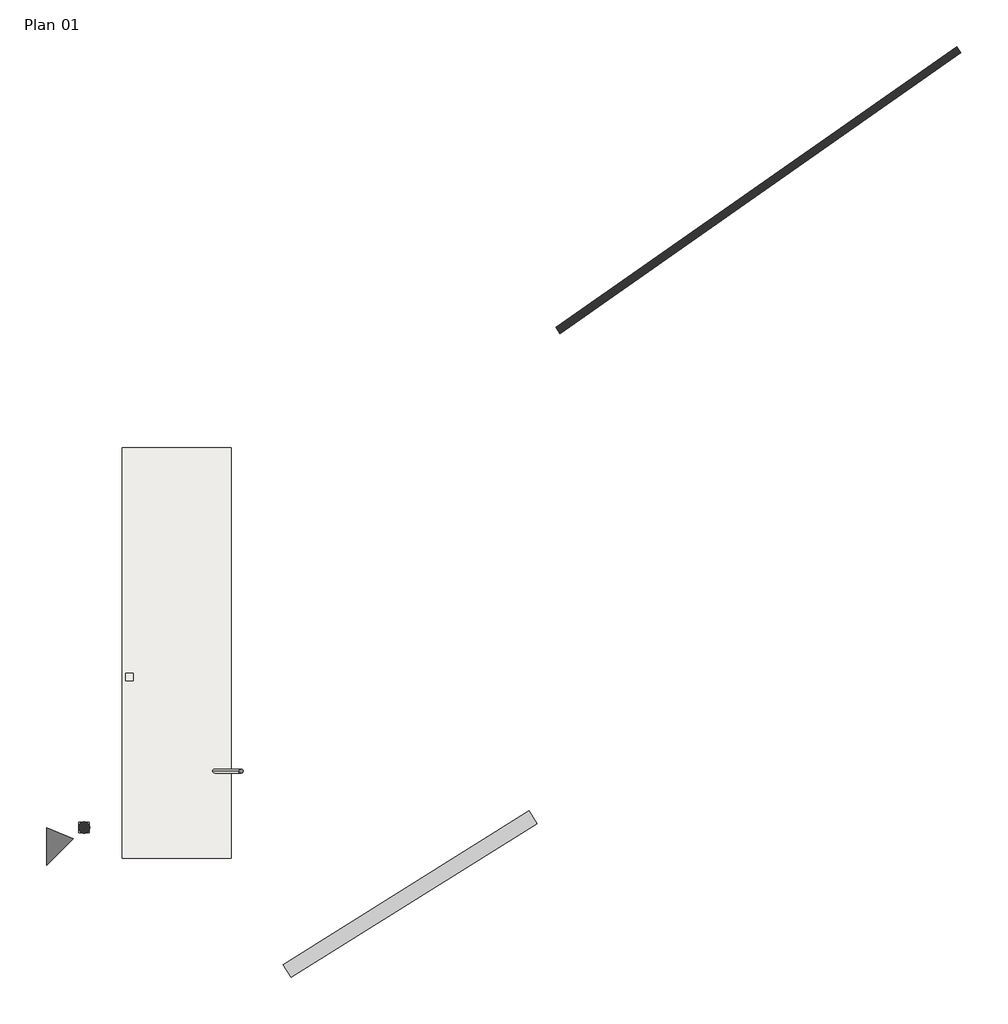
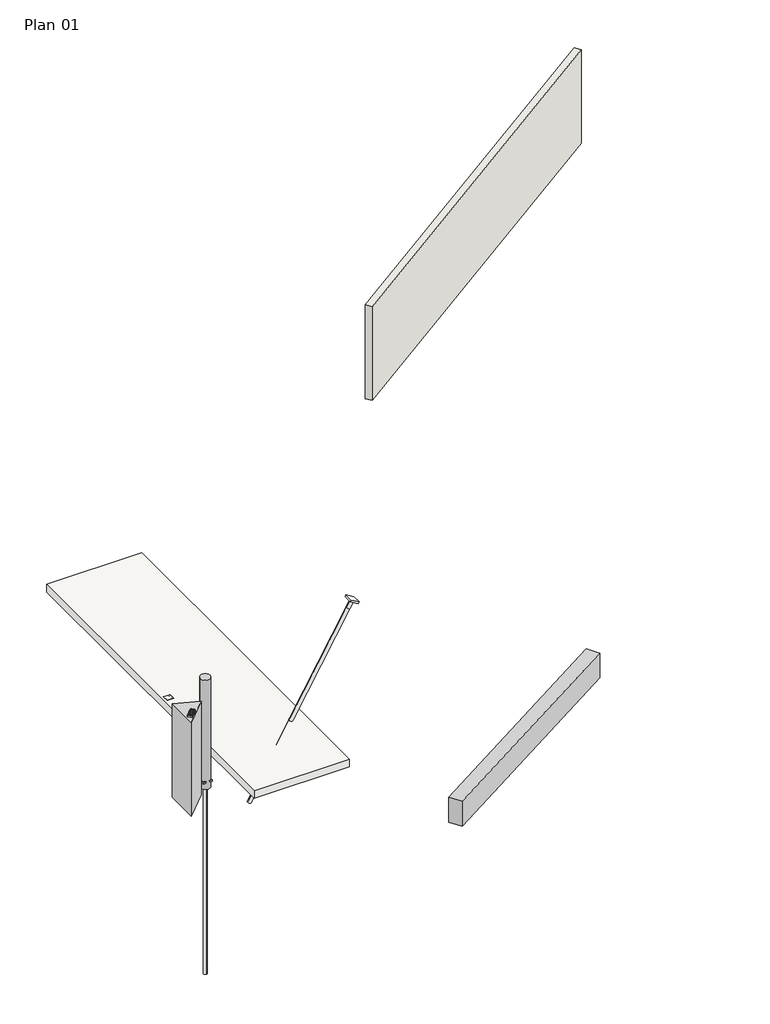
# One storey: 4 slabs, 1 beam, 1 column, 1 geographic element, 1 wall.
"""IFC4 building model written with IfcOpenShell, lengths in millimetres."""

import ifcopenshell
import ifcopenshell.guid

model = None  # the IFC model being written
_history = None  # IfcOwnerHistory: only IFC2X3 demands one
_inside = {}  # id of a spatial element -> (the spatial element, [elements in it])
_under = {}  # id of a project, library or spatial element -> (it, [spatial elements below it])
_declared = {}  # id of a project -> (the project, [libraries it declares])
_typed = {}  # id of a type object -> (the type object, [elements of that type])
_made_of = {}  # id of a material, layer set ... -> (it, [elements and type objects made of it])


def new_model(schema):
    """Start an empty IFC model of exactly this schema.

    Asked for "IFC4X3", IfcOpenShell would pick the latest addendum, in which some entities
    have other attributes; the version numbers below select the first issue.
    IFC2X3 requires an IfcOwnerHistory on every rooted entity: one is made here for all.
    """
    global model, _history
    if schema == "IFC4X3":
        model = ifcopenshell.file(schema_version=(4, 3, 0, 0))
    else:
        model = ifcopenshell.file(schema=schema)
    _inside.clear()
    _under.clear()
    _declared.clear()
    _typed.clear()
    _made_of.clear()
    _history = None
    if model.schema == "IFC2X3":
        org = make("IfcOrganization", Name="unknown")
        user = make(
            "IfcPersonAndOrganization",
            ThePerson=make("IfcPerson", FamilyName="unknown"),
            TheOrganization=org,
        )
        app = make(
            "IfcApplication",
            ApplicationDeveloper=org,
            Version="unknown",
            ApplicationFullName="unknown",
            ApplicationIdentifier="unknown",
        )
        _history = make(
            "IfcOwnerHistory",
            OwningUser=user,
            OwningApplication=app,
            ChangeAction="ADDED",
            CreationDate=0,
        )
    return model


def make(cls, **values):
    """One entity of the class cls with the attributes given. An attribute that is None is left unset."""
    return model.create_entity(
        cls, **{name: value for name, value in values.items() if value is not None}
    )


def rooted(cls, **values):
    """An entity with a GlobalId (a new one), such as an element, a storey or a relation."""
    return make(cls, GlobalId=ifcopenshell.guid.new(), OwnerHistory=_history, **values)


def si_unit(unit_type, name, prefix=None):
    """IfcSIUnit, for example si_unit("LENGTHUNIT", "METRE", prefix="MILLI")."""
    return make("IfcSIUnit", UnitType=unit_type, Prefix=prefix, Name=name)


def assignment(units):
    """IfcUnitAssignment: the units of a project."""
    return None if units is None else make("IfcUnitAssignment", Units=units)


def point(xyz):
    """IfcCartesianPoint."""
    return None if xyz is None else make("IfcCartesianPoint", Coordinates=xyz)


def direction(xyz):
    """IfcDirection."""
    return None if xyz is None else make("IfcDirection", DirectionRatios=xyz)


def frame(location, z_axis=None, x_axis=None):
    """IfcAxis2Placement3D, a coordinate frame: its origin and axes. An axis left out is left unset."""
    return make(
        "IfcAxis2Placement3D",
        Location=point(location),
        Axis=direction(z_axis),
        RefDirection=direction(x_axis),
    )


def frame_2d(location, x_axis=None):
    """IfcAxis2Placement2D, a coordinate frame in the plane: its origin and x axis."""
    return make(
        "IfcAxis2Placement2D", Location=point(location), RefDirection=direction(x_axis)
    )


def origin():
    """The frame at (0, 0, 0) with its axes left unset."""
    return frame((0.0, 0.0, 0.0))


def origin_with_axes():
    """The frame at (0, 0, 0) with the z axis (0, 0, 1) and the x axis (1, 0, 0) written out."""
    return frame((0.0, 0.0, 0.0), z_axis=(0.0, 0.0, 1.0), x_axis=(1.0, 0.0, 0.0))


def origin_2d():
    """The frame at (0, 0) in the plane with its x axis left unset."""
    return frame_2d((0.0, 0.0))


def place(relative_to, where):
    """IfcLocalPlacement: puts the frame where relative to a parent placement (None: the world)."""
    return make(
        "IfcLocalPlacement", PlacementRelTo=relative_to, RelativePlacement=where
    )


def context(
    kind, dimensions, precision=None, world=None, true_north=None, identifier=None
):
    """IfcGeometricRepresentationContext, for example the 3D "Model" context."""
    return make(
        "IfcGeometricRepresentationContext",
        ContextIdentifier=identifier,
        ContextType=kind,
        CoordinateSpaceDimension=dimensions,
        Precision=precision,
        WorldCoordinateSystem=world,
        TrueNorth=true_north,
    )


def project(units=None, contexts=None):
    """IfcProject with its units and contexts."""
    return rooted(
        "IfcProject",
        Name="project",
        RepresentationContexts=contexts,
        UnitsInContext=assignment(units),
    )


def spatial(cls, under=None, at=None, **own):
    """A site, building, storey or space (cls), placed at a placement, below another one or the project."""
    s = rooted(cls, ObjectPlacement=at, **own)
    if under is not None:
        _under.setdefault(under.id(), (under, []))[1].append(s)
    return s


def polyline(points):
    """IfcPolyline through the points."""
    return make("IfcPolyline", Points=[point(p) for p in points])


def circle_curve(where, radius):
    """IfcCircle in the frame where."""
    return make("IfcCircle", Position=where, Radius=radius)


def trimmed(basis, trim1, trim2, sense, master):
    """IfcTrimmedCurve: the piece of a basis curve between two trims."""
    return make(
        "IfcTrimmedCurve",
        BasisCurve=basis,
        Trim1=trim1,
        Trim2=trim2,
        SenseAgreement=sense,
        MasterRepresentation=master,
    )


def segment(curve, same_sense, transition):
    """IfcCompositeCurveSegment."""
    return make(
        "IfcCompositeCurveSegment",
        Transition=transition,
        SameSense=same_sense,
        ParentCurve=curve,
    )


def composite_curve(segments, self_intersect=None):
    """IfcCompositeCurve: segments joined end to end."""
    return make("IfcCompositeCurve", Segments=segments, SelfIntersect=self_intersect)


def outline(outer, holes=None, kind="AREA"):
    """IfcArbitraryClosedProfileDef: a profile drawn as a closed curve; with holes, ...WithVoids."""
    if holes is None:
        return make("IfcArbitraryClosedProfileDef", ProfileType=kind, OuterCurve=outer)
    return make(
        "IfcArbitraryProfileDefWithVoids",
        ProfileType=kind,
        OuterCurve=outer,
        InnerCurves=holes,
    )


def extrude(swept, where, along, depth):
    """IfcExtrudedAreaSolid: the profile swept, set in the frame where, extruded along a direction by depth."""
    return make(
        "IfcExtrudedAreaSolid",
        SweptArea=swept,
        Position=where,
        ExtrudedDirection=direction(along),
        Depth=depth,
    )


def faces_of(points, faces, orient=None, outer=None):
    """IfcFace entities. A face is a list of loops; a loop is a list of indices into points, from 0.

    orient and outer hold one flag for each loop. By default every Orientation is true, the
    first loop of a face is its IfcFaceOuterBound and the others are IfcFaceBound.
    """
    made = []
    for i, loops in enumerate(faces):
        bounds = []
        for j, loop in enumerate(loops):
            is_outer = j == 0 if outer is None else outer[i][j]
            bounds.append(
                make(
                    "IfcFaceOuterBound" if is_outer else "IfcFaceBound",
                    Bound=make("IfcPolyLoop", Polygon=[points[k] for k in loop]),
                    Orientation=True if orient is None else orient[i][j],
                )
            )
        made.append(make("IfcFace", Bounds=bounds))
    return made


def faceted_brep(points, faces, orient=None, outer=None, voids=None):
    """IfcFacetedBrep: a solid bounded by flat faces; with voids (closed shells), ...WithVoids."""
    shared = [point(p) for p in points]
    hull = make("IfcClosedShell", CfsFaces=faces_of(shared, faces, orient, outer))
    if voids is None:
        return make("IfcFacetedBrep", Outer=hull)
    return make(
        "IfcFacetedBrepWithVoids",
        Outer=hull,
        Voids=[
            make(cls, CfsFaces=faces_of(shared, fs, o, b)) for cls, fs, o, b in voids
        ],
    )


def shape(context_of_items, identifier, shape_type, items):
    """IfcShapeRepresentation: the items that make up one representation, for example the "Body"."""
    return make(
        "IfcShapeRepresentation",
        ContextOfItems=context_of_items,
        RepresentationIdentifier=identifier,
        RepresentationType=shape_type,
        Items=items,
    )


def source(mapping_origin, context_of_items, identifier, shape_type, items):
    """IfcRepresentationMap: a shape defined once, which mapped items show again and again."""
    return make(
        "IfcRepresentationMap",
        MappingOrigin=mapping_origin,
        MappedRepresentation=shape(context_of_items, identifier, shape_type, items),
    )


def transform(
    local_origin,
    x_axis=None,
    y_axis=None,
    z_axis=None,
    scale=None,
    scale2=None,
    scale3=None,
    uniform=True,
):
    """IfcCartesianTransformationOperator3D, or its non-uniform kind. x_axis, y_axis, z_axis: its Axis1, 2, 3."""
    if uniform:
        return make(
            "IfcCartesianTransformationOperator3D",
            Axis1=direction(x_axis),
            Axis2=direction(y_axis),
            LocalOrigin=point(local_origin),
            Scale=scale,
            Axis3=direction(z_axis),
        )
    return make(
        "IfcCartesianTransformationOperator3DnonUniform",
        Axis1=direction(x_axis),
        Axis2=direction(y_axis),
        LocalOrigin=point(local_origin),
        Scale=scale,
        Axis3=direction(z_axis),
        Scale2=scale2,
        Scale3=scale3,
    )


def mapped(mapping_source, mapping_target):
    """IfcMappedItem: shows the shape of a source again, moved by a transform."""
    return make(
        "IfcMappedItem", MappingSource=mapping_source, MappingTarget=mapping_target
    )


def made_of(thing, what):
    """Note that an element or type object is made of a material, layer set ...; save() writes the relation."""
    if what is not None:
        _made_of.setdefault(what.id(), (what, []))[1].append(thing)
    return thing


def element(
    cls,
    number,
    at=None,
    inside=None,
    cuts=None,
    type_object=None,
    material=None,
    context=None,
    identifier="Body",
    shape_type=None,
    held_by="IfcProductDefinitionShape",
    body=None,
    shapes=None,
    **own,
):
    """One element of the class cls, such as IfcWall. Its Tag is "e" and its number.

    at: its placement. inside: the storey or other place that contains it. cuts: it is an
    opening in that element (IfcRelVoidsElement). A single representation is given by context,
    identifier, shape_type and body (its items); several are given by shapes. held_by: the class
    of the entity that holds the representations. save() writes the other relations.
    """
    e = rooted(cls, Tag="e%d" % number, ObjectPlacement=at, **own)
    if body is not None:
        shapes = [shape(context, identifier, shape_type, body)]
    if shapes is not None:
        e.Representation = make(held_by, Representations=shapes)
    if inside is not None:
        _inside.setdefault(inside.id(), (inside, []))[1].append(e)
    if cuts is not None:
        rooted(
            "IfcRelVoidsElement", RelatingBuildingElement=cuts, RelatedOpeningElement=e
        )
    if type_object is not None:
        _typed.setdefault(type_object.id(), (type_object, []))[1].append(e)
    return made_of(e, material)


def aggregate(whole, parts):
    """IfcRelAggregates: a whole, such as a stair, and the parts it consists of."""
    return rooted("IfcRelAggregates", RelatingObject=whole, RelatedObjects=parts)


def save(model, path):
    """Write the relations noted so far, then the file.

    IfcRelAggregates (storeys below a building ...), IfcRelContainedInSpatialStructure (elements
    in a storey), IfcRelDefinesByType, IfcRelAssociatesMaterial and IfcRelDeclares: one each for
    every whole, place, type object, material and project.
    """
    for whole, parts in _under.values():
        aggregate(whole, parts)
    for where, things in _inside.values():
        rooted(
            "IfcRelContainedInSpatialStructure",
            RelatedElements=things,
            RelatingStructure=where,
        )
    for kind, things in _typed.values():
        rooted("IfcRelDefinesByType", RelatedObjects=things, RelatingType=kind)
    for what, things in _made_of.values():
        rooted("IfcRelAssociatesMaterial", RelatedObjects=things, RelatingMaterial=what)
    for by, libraries in _declared.values():
        rooted("IfcRelDeclares", RelatingContext=by, RelatedDefinitions=libraries)
    model.write(path)


def plane_surface(at):
    """IfcPlane: the flat surface through the origin of the frame at, square to its z axis."""
    return make("IfcPlane", Position=at)


def cylinder_surface(at, radius):
    """IfcCylindricalSurface: all points at the distance radius from the z axis of the frame at."""
    return make("IfcCylindricalSurface", Position=at, Radius=radius)


def advanced_brep(points, edges, surfaces, faces):
    """IfcAdvancedBrep: a solid bounded by faces that lie on surfaces and meet in shared edges.

    An edge is (start, end): straight between two places in points (the first is 0);
    or (start, end, curve); or (start, end, curve, False) where it runs against its curve.
    A face is (place in surfaces, loops), or (place, loops, False) where it looks against
    its surface's normal. A loop lists edges by number (the first is 1), with a minus sign
    where the edge is run from its end to its start. The first loop is the outer one.
    """
    corners = [point(p) for p in points]
    vertices = [make("IfcVertexPoint", VertexGeometry=c) for c in corners]
    made = []
    for start, end, *more in edges:
        made.append(
            make(
                "IfcEdgeCurve",
                EdgeStart=vertices[start],
                EdgeEnd=vertices[end],
                EdgeGeometry=more[0] if more else make("IfcPolyline", Points=[corners[start], corners[end]]),
                SameSense=more[1] if len(more) > 1 else True,
            )
        )
    hull = []
    for where, loops, *sense in faces:
        bounds = []
        for j, loop in enumerate(loops):
            ring = [make("IfcOrientedEdge", EdgeElement=made[abs(k) - 1], Orientation=k > 0) for k in loop]
            bounds.append(
                make(
                    "IfcFaceOuterBound" if j == 0 else "IfcFaceBound",
                    Bound=make("IfcEdgeLoop", EdgeList=ring),
                    Orientation=True,
                )
            )
        hull.append(make("IfcAdvancedFace", Bounds=bounds, FaceSurface=surfaces[where], SameSense=sense[0] if sense else True))
    return make("IfcAdvancedBrep", Outer=make("IfcClosedShell", CfsFaces=hull))


def beam_400x800mm_1e0f6873(model_context):
    return source(origin(), model_context, "Body", "SweptSolid", [
        extrude(outline(polyline([(3850.0, 200.0), (3850.0, -200.0), (-3850.0, -200.0), (-3850.0, 200.0), (3850.0, 200.0)])), frame((0.0, 0.0, -400.0), z_axis=(0.0, 0.0, 1.0), x_axis=(1.0, 0.0, 0.0)), (0.0, 0.0, 1.0), 800.0),
    ])


def column_bdfed939(model_context):
    return source(origin(), model_context, "Body", "SweptSolid", [
        extrude(outline(composite_curve([segment(trimmed(circle_curve(origin_2d(), 150.0), [point((-150.0, 0.0))], [point((150.0, 0.0))], False, "CARTESIAN"), True, "CONTINUOUS"), segment(trimmed(circle_curve(origin_2d(), 150.0), [point((150.0, 0.0))], [point((-150.0, 0.0))], False, "CARTESIAN"), True, "CONTINUOUS")], self_intersect=False)), origin_with_axes(), (0.0, 0.0, 1.0), 3500.0),
    ])


def rib_79407f03(model_context):
    return source(origin(), model_context, "Body", "SweptSolid", [
        extrude(outline(polyline([(0.0, 1000.0), (707.1067812, 707.1067812), (0.0, 0.0), (0.0, 1000.0)])), origin_with_axes(), (0.0, 0.0, 1.0), 3000.0),
        extrude(outline(polyline([(25.1140775, 0.0), (25.1140775, -200.9126203), (-61.4608186, -200.9126203), (-84.7293549, -199.5575883), (-101.658058, -195.4924922), (-114.0311558, -187.9876995), (-123.6328759, -176.3135776), (-129.7948993, -161.837421), (-131.8489071, -145.9265248), (-128.4459986, -126.1344734), (-118.2372733, -109.7269364), (-100.9161627, -97.6971952), (-76.1760985, -91.0385311), (-90.4499198, -80.2963768), (-110.806057, -54.4465353), (-144.307844, 0.0), (-115.1225391, 0.0), (-88.9783919, -41.6442419), (-70.0937828, -69.210866), (-56.8255055, -82.2338887), (-44.8816034, -87.0163546), (-30.3134764, -87.8992714), (0.0, -87.8992714), (0.0, 0.0), (25.1140775, 0.0)]), holes=[polyline([(0.0, -113.0133489), (-56.2123689, -113.0133489), (-84.882639, -116.5695415), (-94.3126808, -121.1925919), (-101.1675487, -127.9493579), (-106.7348295, -144.994557), (-104.0799478, -157.2450275), (-96.1153027, -167.1165277), (-82.4116983, -173.628039), (-62.5399392, -175.7985428), (0.0, -175.7985428), (0.0, -113.0133489)])]), frame((497.5715471, 793.899117, 2400.0), z_axis=(0.38268343236508784, 0.9238795325112875, 0.0), x_axis=(0.9238795325112875, -0.38268343236508784, 0.0)), (0.0, 0.0, 1.0), 50.0),
        extrude(outline(polyline([(328.1863632, 918.1803674), (351.3887454, 908.569626), (332.2545738, 862.3756494), (309.0521916, 871.9863908), (328.1863632, 918.1803674)])), frame((0.0, 0.0, 2400.0), z_axis=(0.0, 0.0, 1.0), x_axis=(1.0, 0.0, 0.0)), (0.0, 0.0, 1.0), 200.9126203),
        extrude(outline(polyline([(76.0779965, 0.0), (76.0779965, -200.9126203), (-0.5886112, -200.9126203), (-21.6743809, -199.434961), (-38.1371002, -195.0019829), (-50.7554526, -187.5033216), (-60.3081217, -176.8286123), (-66.3229924, -164.2715736), (-68.3279493, -151.1259236), (-66.6418234, -139.0287373), (-61.583446, -127.6550523), (-53.1160287, -117.7038444), (-41.2027834, -109.8740892), (-55.4336854, -102.4428729), (-65.948979, -91.1366329), (-72.4420962, -76.703396), (-74.6064686, -59.8911888), (-68.6958312, -32.8886504), (-54.0541278, -13.6606848), (-32.2019373, -3.4580908), (0.0, 0.0), (76.0779965, 0.0)]), holes=[polyline([(50.9639191, -119.2918683), (5.101297, -119.2918683), (-21.6805123, -121.4501093), (-37.7937437, -130.7452611), (-43.2138717, -147.1037471), (-38.1616256, -163.4867587), (-23.6916005, -173.1743179), (8.5839132, -175.7985428), (50.9639191, -175.7985428), (50.9639191, -119.2918683)]), polyline([(50.9639191, -25.1140775), (-0.5395603, -25.1140775), (-19.1789147, -26.0950962), (-34.9487895, -31.5642752), (-45.3966382, -42.7233624), (-49.4923911, -59.6459342), (-44.6853997, -79.1682054), (-38.3884862, -86.2254083), (-29.1117286, -90.8178019), (1.9129864, -94.1777908), (50.9639191, -94.1777908), (50.9639191, -25.1140775)])]), frame((192.3605232, 920.3216624, 2400.0), z_axis=(0.38268343236508784, 0.9238795325112875, 0.0), x_axis=(0.9238795325112875, -0.38268343236508784, 0.0)), (0.0, 0.0, 1.0), 50.0),
        extrude(outline(polyline([(142.0846737, 166.9156415), (34.8288922, 272.7551681), (80.4360125, 318.9725642), (104.5051668, 337.5762862), (115.0296187, 340.2280985), (126.319893, 339.2040535), (137.2940026, 334.8676564), (146.8699607, 327.5824121), (155.6431762, 315.3394631), (159.0243303, 301.2462182), (156.3216686, 285.6622725), (146.8434364, 268.9472211), (160.0974204, 270.9082992), (184.6206627, 268.1577423), (231.3350949, 257.3603361), (215.9604566, 241.7799674), (179.9563975, 249.7610286), (155.2918548, 254.2015408), (141.3499598, 253.9788127), (132.5049003, 250.1220185), (124.3591622, 242.810042), (108.3902102, 226.627407), (155.3146145, 180.3226141), (142.0846737, 166.9156415)]), holes=[polyline([(94.9832375, 239.8573479), (124.595566, 269.8659235), (137.8004388, 287.0447247), (140.3041941, 301.7331255), (134.1375442, 313.6844846), (126.1991419, 318.7206668), (116.7335855, 319.6690426), (106.0384872, 315.7836943), (94.4114592, 306.3187042), (61.4658058, 272.9322), (94.9832375, 239.8573479)])]), frame((0.0, 0.0, 3000.0), z_axis=(0.0, 0.0, 1.0), x_axis=(1.0, 0.0, 0.0)), (0.0, 0.0, 1.0), 50.0),
        extrude(outline(polyline([(249.577943, 275.8472945), (142.3221615, 381.6868212), (155.5521023, 395.0937938), (262.8078838, 289.2542672), (249.577943, 275.8472945)])), frame((0.0, 0.0, 3000.0), z_axis=(0.0, 0.0, 1.0), x_axis=(1.0, 0.0, 0.0)), (0.0, 0.0, 1.0), 50.0),
        extrude(outline(polyline([(289.2677655, 316.0682125), (182.011984, 421.9077392), (222.3994792, 462.8356656), (245.3351431, 479.7669736), (255.9855205, 482.5529434), (266.7164256, 482.0291974), (284.6624197, 472.770508), (293.6392157, 456.8056927), (292.3950501, 436.5587187), (303.8589035, 440.2410662), (315.4340515, 439.898524), (326.559667, 435.7614887), (336.6749229, 428.0603568), (347.9763498, 410.6802344), (350.5279044, 392.7346911), (344.4628882, 375.6943903), (329.3451839, 356.681913), (289.2677655, 316.0682125)]), holes=[polyline([(238.8145861, 392.3174042), (262.9747319, 416.8008406), (275.9310618, 432.2350681), (279.4572615, 445.7336312), (273.5796894, 457.2446776), (262.1722425, 463.178041), (249.3778877, 460.5566667), (230.9744227, 444.7090375), (208.6488975, 422.0847711), (238.8145861, 392.3174042)]), polyline([(289.0907336, 342.7051261), (316.2224482, 370.1998943), (325.5178351, 380.6671764), (330.9056251, 391.9669422), (330.4522875, 403.4229905), (323.5759095, 414.5241854), (310.6217897, 422.2422189), (296.1986213, 420.0652601), (278.0612869, 405.2729569), (252.2215587, 379.0874633), (289.0907336, 342.7051261)])]), frame((0.0, 0.0, 3000.0), z_axis=(0.0, 0.0, 1.0), x_axis=(1.0, 0.0, 0.0)), (0.0, 0.0, 1.0), 50.0),
    ])


def slab_200x200_02b47a6d(model_context):
    return source(origin(), model_context, "Body", "SweptSolid", [
        extrude(outline(composite_curve([segment(trimmed(circle_curve(frame_2d((269.1096391, -214.6158832)), 6.0), [point((263.1096391, -214.6158832))], [point((275.1096391, -214.6158832))], False, "CARTESIAN"), True, "CONTINUOUS"), segment(trimmed(circle_curve(frame_2d((269.1096391, -214.6158832)), 6.0), [point((275.1096391, -214.6158832))], [point((263.1096391, -214.6158832))], False, "CARTESIAN"), True, "CONTINUOUS")], self_intersect=False)), frame((0.0, 0.0, -200.0), z_axis=(0.0, 0.0, 1.0), x_axis=(1.0, 0.0, 0.0)), (0.0, 0.0, 1.0), 185.0),
        extrude(outline(composite_curve([segment(trimmed(circle_curve(frame_2d((369.1096391, -214.6158832)), 6.0), [point((363.1096391, -214.6158832))], [point((375.1096391, -214.6158832))], False, "CARTESIAN"), True, "CONTINUOUS"), segment(trimmed(circle_curve(frame_2d((369.1096391, -214.6158832)), 6.0), [point((375.1096391, -214.6158832))], [point((363.1096391, -214.6158832))], False, "CARTESIAN"), True, "CONTINUOUS")], self_intersect=False)), frame((0.0, 0.0, -200.0), z_axis=(0.0, 0.0, 1.0), x_axis=(1.0, 0.0, 0.0)), (0.0, 0.0, 1.0), 185.0),
        extrude(outline(composite_curve([segment(trimmed(circle_curve(frame_2d((369.1096391, -314.6158832)), 6.0), [point((363.1096391, -314.6158832))], [point((375.1096391, -314.6158832))], False, "CARTESIAN"), True, "CONTINUOUS"), segment(trimmed(circle_curve(frame_2d((369.1096391, -314.6158832)), 6.0), [point((375.1096391, -314.6158832))], [point((363.1096391, -314.6158832))], False, "CARTESIAN"), True, "CONTINUOUS")], self_intersect=False)), frame((0.0, 0.0, -200.0), z_axis=(0.0, 0.0, 1.0), x_axis=(1.0, 0.0, 0.0)), (0.0, 0.0, 1.0), 185.0),
        extrude(outline(composite_curve([segment(trimmed(circle_curve(frame_2d((269.1096391, -314.6158832)), 6.0), [point((263.1096391, -314.6158832))], [point((275.1096391, -314.6158832))], False, "CARTESIAN"), True, "CONTINUOUS"), segment(trimmed(circle_curve(frame_2d((269.1096391, -314.6158832)), 6.0), [point((275.1096391, -314.6158832))], [point((263.1096391, -314.6158832))], False, "CARTESIAN"), True, "CONTINUOUS")], self_intersect=False)), frame((0.0, 0.0, -200.0), z_axis=(0.0, 0.0, 1.0), x_axis=(1.0, 0.0, 0.0)), (0.0, 0.0, 1.0), 185.0),
        extrude(outline(polyline([(419.1096391, -164.6158832), (419.1096391, -364.6158832), (219.1096391, -364.6158832), (219.1096391, -164.6158832), (419.1096391, -164.6158832)])), frame((0.0, 0.0, -15.0), z_axis=(0.0, 0.0, 1.0), x_axis=(1.0, 0.0, 0.0)), (0.0, 0.0, 1.0), 15.0),
    ])


model = new_model("IFC4")

# Units and contexts
model_context = context("Model", 3, world=origin())
ifc_project = project(units=[si_unit("LENGTHUNIT", "METRE", prefix="MILLI")], contexts=[model_context])

# Site, building, storey
site = spatial("IfcSite", under=ifc_project)
building = spatial("IfcBuilding", under=site)
storey = spatial("IfcBuildingStorey", under=building, Name="Plan 01", Elevation=0.0)

# Beam
placement = place(None, origin())
beam_400x800mm_shape = beam_400x800mm_1e0f6873(model_context)
element("IfcBeam", 1, ObjectType="S-Frame_CastInPlace_Rectangular : 400x800mm", at=placement, inside=storey, context=model_context, shape_type="MappedRepresentation", body=[
    mapped(beam_400x800mm_shape, transform((9658.2803674, -768.6963803, -400.0), x_axis=(0.8480480961564263, 0.5299192642332045, 0.0), y_axis=(-0.5299192642332045, 0.8480480961564263, 0.0), z_axis=(0.0, 0.0, 1.0))),
])

# Column
column_shape = column_bdfed939(model_context)
element("IfcColumn", 2, ObjectType="S-Column_CastInPlace_Round : Ø300", at=placement, inside=storey, context=model_context, shape_type="MappedRepresentation", body=[
    mapped(column_shape, transform((1000.0, 1000.0, 0.0), x_axis=(1.0, 0.0, 0.0), y_axis=(0.0, 1.0, 0.0), z_axis=(0.0, 0.0, 1.0))),
])

# Geographic element
rib_shape = rib_79407f03(model_context)
element("IfcGeographicElement", 3, ObjectType="NO_Origo : RIB", at=placement, inside=storey, context=model_context, shape_type="MappedRepresentation", body=[
    mapped(rib_shape, transform((0.0, 0.0, 0.0), x_axis=(1.0, 0.0, 0.0), y_axis=(0.0, 1.0, 0.0), z_axis=(0.0, 0.0, 1.0))),
])

# Slabs
element("IfcSlab", 4, ObjectType="Betongdekke 250mm", at=placement, inside=storey, context=model_context, shape_type="Brep", body=[
    faceted_brep([(2011.4794189, 11088.1813587, -250.0), (4900.8131513, 11088.1813587, -250.0), (4900.8131513, 182.737712, -250.0), (2011.4794189, 182.737712, -250.0), (4900.8131513, 11088.1813587, 0.0), (2011.4794189, 11088.1813587, 0.0), (2011.4794189, 182.737712, 0.0), (4900.8131513, 182.737712, 0.0), (2300.0, 4900.0, 0.0), (2100.0, 4900.0, 0.0), (2100.0, 5100.0, 0.0), (2300.0, 5100.0, 0.0), (2100.0, 4900.0, -15.0), (2300.0, 4900.0, -15.0), (2300.0, 5100.0, -15.0), (2100.0, 5100.0, -15.0)], [[[0, 1, 2, 3]], [[4, 5, 6, 7], [8, 9, 10, 11]], [[1, 0, 5, 4]], [[2, 1, 4, 7]], [[3, 2, 7, 6]], [[0, 3, 6, 5]], [[12, 13, 14, 15]], [[13, 12, 9, 8]], [[14, 13, 8, 11]], [[15, 14, 11, 10]], [[12, 15, 10, 9]]]),
])
slab_200x200_shape = slab_200x200_02b47a6d(model_context)
element("IfcSlab", 5, ObjectType="Innstøpningsplate : 200x200", at=placement, inside=storey, context=model_context, shape_type="MappedRepresentation", body=[
    mapped(slab_200x200_shape, transform((2519.1096391, 4735.3841168, 0.0), x_axis=(-1.0, 0.0, 0.0), y_axis=(0.0, -1.0, 0.0), z_axis=(0.0, 0.0, 1.0))),
])
element("IfcSlab", 6, ObjectType="Pel-ST : D110T", at=placement, inside=storey, context=model_context, shape_type="SolidModel", body=[
    advanced_brep(
    [(6363.101451, 2500.0, 3172.5), (6267.8386566, 2500.0, 3227.5), (6152.3686028, 2500.0, 3027.5), (6247.6313972, 2500.0, 2972.5), (3247.6313972, 2500.0, -2223.6524227), (3152.3686028, 2500.0, -2168.6524227)],
    [
        (0, 1, circle_curve(frame((6315.4700538, 2500.0, 3200.0), z_axis=(0.499999999999998, 0.0, 0.8660254037844398), x_axis=(-0.8660254037844398, 0.0, 0.499999999999998)), 55.0)),
        (1, 0, circle_curve(frame((6315.4700538, 2500.0, 3200.0), z_axis=(0.499999999999998, 0.0, 0.8660254037844398), x_axis=(-0.8660254037844398, 0.0, 0.499999999999998)), 55.0)),
        (1, 2),
        (2, 3, circle_curve(frame((6200.0, 2500.0, 3000.0), z_axis=(0.499999999999998, 0.0, 0.8660254037844398), x_axis=(-0.8660254037844398, 0.0, 0.499999999999998)), 55.0)),
        (3, 0),
        (3, 2, circle_curve(frame((6200.0, 2500.0, 3000.0), z_axis=(0.499999999999998, 0.0, 0.8660254037844398), x_axis=(-0.8660254037844398, 0.0, 0.499999999999998)), 55.0)),
        (4, 5, circle_curve(frame((3200.0, 2500.0, -2196.1524227), z_axis=(-0.49999999999999933, 0.0, -0.866025403784439), x_axis=(-0.866025403784439, 0.0, 0.49999999999999933)), 55.0)),
        (5, 4, circle_curve(frame((3200.0, 2500.0, -2196.1524227), z_axis=(-0.49999999999999933, 0.0, -0.866025403784439), x_axis=(-0.866025403784439, 0.0, 0.49999999999999933)), 55.0)),
        (2, 5),
        (4, 3),
    ],
    [
        plane_surface(frame((6315.4700538, 2500.0, 3200.0), z_axis=(0.49999999999999806, 0.0, 0.8660254037844398), x_axis=(0.0, 1.0, 0.0))),
        cylinder_surface(frame((6315.4700538, 2500.0, 3200.0), z_axis=(0.499999999999998, 0.0, 0.8660254037844398), x_axis=(-0.8660254037844398, 0.0, 0.499999999999998)), 55.0),
        plane_surface(frame((3200.0, 2500.0, -2196.1524227), z_axis=(-0.49999999999999944, 0.0, -0.866025403784439), x_axis=(0.0, 1.0, 0.0))),
        cylinder_surface(frame((6200.0, 2500.0, 3000.0), z_axis=(0.49999999999999933, 0.0, 0.866025403784439), x_axis=(-0.866025403784439, 0.0, 0.49999999999999933)), 55.0),
    ],
    [
        (0, [[1, 2]]),
        (1, [[-2, 3, 4, 5]]),
        (1, [[-1, -5, 6, -3]]),
        (2, [[7, 8]]),
        (3, [[-4, 9, -7, 10]]),
        (3, [[-6, -10, -8, -9]]),
    ],
),
    extrude(outline(polyline([(280.0, 0.0), (280.0, -280.0), (0.0, -280.0), (0.0, 0.0), (280.0, 0.0)])), frame((6436.7136104, 2360.0, 3130.0), z_axis=(0.49999999999999806, 0.0, 0.8660254037844398), x_axis=(-0.8660254037844398, 0.0, 0.49999999999999806)), (0.0, 0.0, 1.0), 50.0),
])
element("IfcSlab", 7, ObjectType="Pel-ST : D110T", at=placement, inside=storey, context=model_context, shape_type="SolidModel", body=[
    extrude(outline(polyline([(1140.0, 1140.0), (1140.0, 860.0), (860.0, 860.0), (860.0, 1140.0), (1140.0, 1140.0)])), frame((0.0, 0.0, 200.0), z_axis=(0.0, 0.0, 1.0), x_axis=(1.0, 0.0, 0.0)), (0.0, 0.0, 1.0), 50.0),
    advanced_brep(
    [(1000.0, 1055.0, 200.0), (1000.0, 945.0, 200.0), (1000.0, 1055.0, 0.0), (1000.0, 945.0, 0.0), (1000.0, 1055.0, -6000.0), (1000.0, 945.0, -6000.0)],
    [
        (0, 1, circle_curve(frame((1000.0, 1000.0, 200.0), z_axis=(0.0, 0.0, 1.0), x_axis=(0.0, -1.0, 0.0)), 55.0)),
        (1, 0, circle_curve(frame((1000.0, 1000.0, 200.0), z_axis=(0.0, 0.0, 1.0), x_axis=(0.0, -1.0, 0.0)), 55.0)),
        (0, 2),
        (2, 3, circle_curve(frame((1000.0, 1000.0, 0.0), z_axis=(0.0, 0.0, 1.0), x_axis=(0.0, -1.0, 0.0)), 55.0)),
        (3, 1),
        (3, 2, circle_curve(frame((1000.0, 1000.0, 0.0), z_axis=(0.0, 0.0, 1.0), x_axis=(0.0, -1.0, 0.0)), 55.0)),
        (4, 5, circle_curve(frame((1000.0, 1000.0, -6000.0), z_axis=(0.0, 0.0, -1.0), x_axis=(0.0, -1.0, 0.0)), 55.0)),
        (5, 4, circle_curve(frame((1000.0, 1000.0, -6000.0), z_axis=(0.0, 0.0, -1.0), x_axis=(0.0, -1.0, 0.0)), 55.0)),
        (2, 4),
        (5, 3),
    ],
    [
        plane_surface(frame((1000.0, 1000.0, 200.0), z_axis=(0.0, 0.0, 1.0), x_axis=(0.0, -1.0, 0.0))),
        cylinder_surface(frame((1000.0, 1000.0, 200.0), z_axis=(0.0, 0.0, 1.0), x_axis=(0.0, -1.0, 0.0)), 55.0),
        plane_surface(frame((1000.0, 1000.0, -6000.0), z_axis=(0.0, 0.0, -1.0), x_axis=(0.0, -1.0, 0.0))),
        cylinder_surface(frame((1000.0, 1000.0, 0.0), z_axis=(0.0, 0.0, 1.0), x_axis=(0.0, -1.0, 0.0)), 55.0),
    ],
    [
        (0, [[1, 2]]),
        (1, [[-1, 3, 4, 5]]),
        (1, [[-2, -5, 6, -3]]),
        (2, [[7, 8]]),
        (3, [[-4, 9, -8, 10]]),
        (3, [[-6, -10, -7, -9]]),
    ],
),
])

# Wall
element("IfcWall", 8, ObjectType="IV Betong 200", at=placement, inside=storey, context=model_context, shape_type="SweptSolid", body=[
    extrude(outline(polyline([(24288.3229054, 21569.8599248), (13639.3463296, 14113.3662523), (13524.6310424, 14277.1966611), (24173.6076181, 21733.6903337), (24288.3229054, 21569.8599248)])), origin_with_axes(), (0.0, 0.0, 1.0), 3000.0),
])

save(model, "model.ifc")

# Revit data of these elements
# Project information
#   Rebar Schedule Template = "K:\\Autodesk\\2020\\Revit\\Apps\\ISY CAD Rebar\\RebarTemplate\\RebarTemplateNOR.docx"
#   Rebar Schedule Sum Template = "K:\\Autodesk\\2020\\Revit\\Apps\\ISY CAD Rebar\\RebarTemplate\\SummationTemplateNOR.docx"
#   Building Name = "Byggets navn"
#   IfcSite GUID = "26J_F9IST8JeFlb3VaP2d$"
#   IfcBuilding GUID = "26J_F9IST8JeFlb3VaP2dy"
#   IfcProject GUID = "26J_F9IST8JeFlb3VaP2dz"
#   SiteName = "Tomtens navn"
#   IfcName = "Prosjektets navn"
#   BIM koordinator = "initialer"
#   Project Issue Date = "Issue Date"
#   Project Status = "Project Status"
#   Client Name = "Kunde"
#   Project Address = "Enter address here"
#   Project Name = "Project Name"
#   Project Number = "523XXXXX"
#   SR Document GUID = "163d8f55-bdac-4b06-afa0-7601cb1705ab"
# Grids (mm)
#   "1": line (10000, 28123.377) -> (10000, 5703.719)
#   "A": line (29560.591, 10000) -> (4962.505, 10000)
# Type "S-Frame_CastInPlace_Rectangular : 400x800mm"
#   NS3457-8 Code = "ABA"
#   NS3451 Code = "2230"
#   NS3457-8 = "ABA Konstruktive bjelker"
#   NS3451 = "2230 Bjelker"
#   ModelBy = "Norconsult AS"
#   Manufacturer = "Norconsult"
#   Width = 400 mm
#   Height = 800 mm
#   Length [instance default] = 1524 mm
#   Structural Material = NO_Betong - Plasstøpt
#   Assembly Code = ""
# Type "S-Column_CastInPlace_Round : Ø300"
#   NS3457-8 Code = "ASA"
#   NS3451 Code = "2220"
#   NS3457-8 = "ASA Konstruktive søyler"
#   NS3451 = "2220 Søyler"
#   Manufacturer = "Norconsult"
#   Description = "Plasstøpt"
#   Diameter = 300 mm
#   Structural Material = Concrete - Cast In Place
#   Assembly Code = ""
# Type "NO_Origo : RIB"
#   Manufacturer = "Norconsult"
#   Text Height = 400 mm
#   Sill Height = 0 mm
#   Height3 = 1000 mm
#   Height = 3000 mm
#   SITE = no
#   RIVv = no
#   RIVr = no
#   RIV = no
#   RISt = no
#   RIPre = no
#   RIMEK = no
#   RIG = no
#   RIE = no
#   RIBr = no
#   RIB = yes
#   LARK = no
#   ARK = no
#   Top Material = none
#   Material = none
#   Assembly Code = ""
# Type "Betongdekke 250mm"
#   Type Comments = "250"
#   Description = "Betongdekke"
#   NS3457-8 Code = "ADA"
#   NS3451 Code = "2510"
#   NS3457-8 = "ADA Konstruktive dekker"
#   NS3451 = "2510 Frittbærende dekker"
#   Function = 0
#   Layers, outside or top first: 250 mm "NO_Betong - Plasstøpt" (function 1)
# Type "Innstøpningsplate : 200x200"
#   NS3457-8 Code = "BAD"
#   NS3451 Code = ""
#   NS3457-8 = "BAD Knutepunkt, innstøpningsgods"
#   NS3451 = ""
#   Manufacturer = "Norconsult"
#   T = 15 mm
#   H = 200 mm
#   Default Elevation = 1000 mm
#   B = 200 mm
#   Armering d = 200 mm
#   Armering b = 50 mm
#   Armering Radius = 6 mm
#   Armering Dia = 12 mm
#   Material Plate = Metal - Steel - 345 MPa
#   Material Armering = Metal - Steel - 345 MPa
#   Assembly Code = ""
# Type "Pel-ST : D110T"
#   NS3457-8 Code = "AHA"
#   NS3451 Code = "2150"
#   NS3457-8 = "AHA Peler"
#   NS3451 = "2150 Pelefundamentering"
#   Toleranser = "+/-50mm"
#   Manufacturer = "Norconsult"
#   Description = "ST-pel"
#   Vekt = 74.6
#   Trykkapasitet = 2194
#   Strekkplate Tykkelse = 10 mm
#   PileLenght [instance default] = 6000 mm
#   PileHead_Thickness = 50 mm
#   Minimum Innstøpning [instance default] = 200 mm
#   Radius = 55 mm
#   Strekkplate Høyde = 140 mm
#   Forankringslengde Fjell [instance default] = 0 mm
#   Dybde [instance default] = 6000 mm
#   Strekkplate Bredde = 142.99 mm
#   PileHead_Lenght = 280 mm
#   Default Elevation = 1000 mm
#   D = 110 mm
#   Angle [instance default] = 0.00°
#   Structural Material = NO_Metall - Stål
#   Kraft = element 654940
#   URL = ""
#   Type Comments = ""
#   Assembly Code = ""
# Type "IV Betong 200"
#   Description = "Betongvegger"
#   NS3457-8 Code = "AVB"
#   NS3451 Code = "2410"
#   NS3457-8 = "AVB Konstruktive innervegger"
#   NS3451 = "2410 Bærende innervegger"
#   Layers, outside or top first: 200 mm "NO_Betong - Plasstøpt" (function 1)
# Element 1 (IfcBeam, "S-Frame_CastInPlace_Rectangular : 400x800mm")
#   Comments = "400x800mm"
#   Phase Created = New Construction
#   Materials on its faces: "NO_Betong - Plasstøpt"
# Element 2 (IfcColumn, "S-Column_CastInPlace_Round : Ø300")
#   Comments = "Ø300"
#   Phase Created = New Construction
#   Materials on its faces: "Concrete - Cast In Place"
# Element 3 (IfcGeographicElement, "NO_Origo : RIB")
#   IfcGUID = "1EH6FudmT63O$f0KliAMRA"
#   Phase Created = New Construction
#   Materials on its faces: "RIB"
# Element 4 (IfcSlab, "Betongdekke 250mm")
#   Comments = ""
#   built-in parameter 1001955 = 3.14159 (stored number, unit not read)
#   Height Offset From Level = 0 mm
#   built-in parameter 1001954 = 1
#   Phase Created = New Construction
#   Materials on its faces: "NO_Betong - Plasstøpt"
# Element 5 (IfcSlab, "Innstøpningsplate : 200x200")
#   Phase Created = New Construction
#   Materials on its faces: "Metal - Steel - 345 MPa"
# Element 6 (IfcSlab, "Pel-ST : D110T")
#   PileLenght = 6000 mm
#   Minimum Innstøpning = 200 mm
#   Forankringslengde Fjell = 0 mm
#   Dybde = 6000 mm
#   Angle = 30.00°
#   Phase Created = New Construction
#   Materials on its faces: "NO_Metall - Stål"
# Element 7 (IfcSlab, "Pel-ST : D110T")
#   Mark = "3"
#   PileLenght = 6000 mm
#   Minimum Innstøpning = 200 mm
#   Forankringslengde Fjell = 0 mm
#   Dybde = 6000 mm
#   Angle = 0.00°
#   Phase Created = New Construction
#   Materials on its faces: "NO_Metall - Stål"
# Element 8 (IfcWall, "IV Betong 200")
#   Comments = "IV Betong 200"
#   Top Offset = 0 mm
#   Base Offset = 0 mm
#   Unconnected Height = 3000 mm
#   wall height = 3000 mm
#   Phase Created = New Construction
#   Base Constraint = Plan 01
#   Materials on its faces: "NO_Betong - Plasstøpt"
# Materials
#   "NO_Betong - Plasstøpt": class "Betong", colour RGB 186 186 186, transparency 0, Material PI-Name = "Betong B45. 120 kg armering pr m3 betong. Lavkarbonklasse B", Cost = 0, Material CO2e = 230.00 kg/m³
#   "Concrete - Cast In Place": class "Concrete", colour RGB 186 186 186, transparency 0, Cost = 0
#   "Metal - Steel - 345 MPa": class "Unassigned", colour RGB 128 64 64, transparency 0, Description = "Steel 345 MPa"
#   "NO_Metall - Stål": class "Metall", colour RGB 128 0 0, transparency 0, Cost = 0
#   "RIB": class "Unassigned", colour RGB 0 255 0, transparency 0, Description = "Dummy material", Cost = 0
